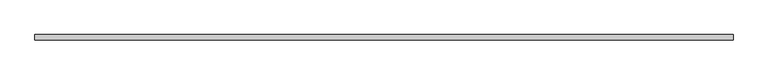
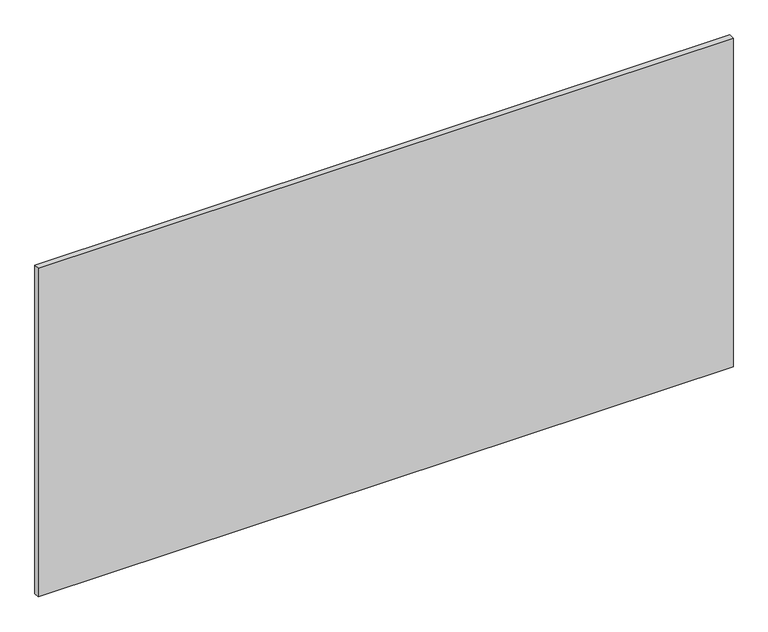
"""IFC4 building model written with IfcOpenShell, lengths in millimetres: proxy geometry, Inner panel:Inner panel:1:Inner panel:1 : Inner panel:Inner panel:300324:300043:Inner panel:1:Inner panel:1 : Inner panel:Inner panel:300324:300043 : Inner panel:Inner panel:1:Inner panel:1 : Inner panel:Inner panel:300324:300043:25 : Inner panel:Inner panel:1:Inner panel:1 : Inner panel:Inner panel:300324:300043:Inner panel:1:Inner panel:1 : Inner panel:Inner panel:300324:300043 : Inner panel:Inner panel:1:Inner panel:1 : Inner panel:Inner panel:300324:300043:300031."""

from ifc_helpers import new_model, si_unit, frame, origin, place, context, project, spatial, polyline, outline, extrude, source, transform, mapped, element, save


def generic_models_4a509fb6(model_context):
    return source(origin(), model_context, "Body", "SweptSolid", [
        extrude(outline(polyline([(592512.5367239, -567913.5913841), (594950.9367239, -567913.5913841), (594950.9367239, -567932.6413841), (592512.5367239, -567932.6413841), (592512.5367239, -567913.5913841)])), frame((0.0, 0.0, 3721.1), z_axis=(0.0, 0.0, 1.0), x_axis=(1.0, 0.0, 0.0)), (0.0, 0.0, 1.0), 1219.2),
    ])


if __name__ == "__main__":
    model = new_model("IFC4")
    model_context = context("Model", 3, world=origin())
    ifc_project = project(units=[si_unit("LENGTHUNIT", "METRE", prefix="MILLI")], contexts=[model_context])
    site = spatial("IfcSite", under=ifc_project)
    building = spatial("IfcBuilding", under=site)
    placement = place(None, origin())
    generic_models_shape = generic_models_4a509fb6(model_context)
    element("IfcBuildingElementProxy", 1, Name="Inner panel:Inner panel:1:Inner panel:1 : Inner panel:Inner panel:300324:300043:Inner panel:1:Inner panel:1 : Inner panel:Inner panel:300324:300043 : Inner panel:Inner panel:1:Inner panel:1 : Inner panel:Inner panel:300324:300043:25 : Inner panel:Inner panel:1:Inner panel:1 : Inner panel:Inner panel:300324:300043:Inner panel:1:Inner panel:1 : Inner panel:Inner panel:300324:300043 : Inner panel:Inner panel:1:Inner panel:1 : Inner panel:Inner panel:300324:300043:300031", ObjectType="Inner panel:Inner panel:1:Inner panel:1 : Inner panel:Inner panel:300324:300043:Inner panel:1:Inner panel:1 : Inner panel:Inner panel:300324:300043 : Inner panel:Inner panel:1:Inner panel:1 : Inner panel:Inner panel:300324:300043:25 : Inner panel:Inner panel:1:Inner panel:1 : Inner panel:Inner panel:300324:300043:Inner panel:1:Inner panel:1 : Inner panel:Inner panel:300324:300043 : Inner panel:Inner panel:1:Inner panel:1 : Inner panel:Inner panel:300324:300043:300031", at=placement, inside=building, context=model_context, shape_type="MappedRepresentation", body=[
        mapped(generic_models_shape, transform((0.0, 0.0, 0.0), x_axis=(1.0, 0.0, 0.0), y_axis=(0.0, 1.0, 0.0), z_axis=(0.0, 0.0, 1.0))),
    ])
    save(model, "model.ifc")

# Revit data of these elements
# Type "Inner panel:Inner panel:1:Inner panel:1 : Inner panel:Inner panel:300324:300043:Inner panel:1:Inner panel:1 : Inner panel:Inner panel:300324:300043 : Inner panel:Inner panel:1:Inner panel:1 : Inner panel:Inner panel:300324:300043:25 : Inner panel:Inner panel:1:Inner panel:1 : Inner panel:Inner panel:300324:300043:Inner panel:1:Inner panel:1 : Inner panel:Inner panel:300324:300043 : Inner panel:Inner panel:1:Inner panel:1 : Inner panel:Inner panel:300324:300043:300031"
#   NameOverride = "Inner panel:Inner panel:1:Inner panel:1 : Inner panel:Inner panel:300324:300043:Inner panel:1:Inner panel:1 : Inner panel:Inner panel:300324:300043 : Inner panel:Inner panel:1:Inner panel:1 : Inner panel:Inner panel:300324:300043:300031"
#   ObjectTypeOverride = "Inner panel:1:Inner panel:1 : Inner panel:Inner panel:300324:300043 : Inner panel:Inner panel:1:Inner panel:1 : Inner panel:Inner panel:300324:300043"
#   Reference = "Inner panel"
#   Tag = "300031"
# Element 1 (IfcBuildingElementProxy, "Inner panel:Inner panel:1:Inner panel:1 : Inner panel:Inner panel:300324:300043:Inner panel:1:Inner panel:1 : Inner panel:Inner panel:300324:300043 : Inner panel:Inner panel:1:Inner panel:1 : Inner panel:Inner panel:300324:300043:25 : Inner panel:Inner panel:1:Inner panel:1 : Inner panel:Inner panel:300324:300043:Inner panel:1:Inner panel:1 : Inner panel:Inner panel:300324:300043 : Inner panel:Inner panel:1:Inner panel:1 : Inner panel:Inner panel:300324:300043:300031")
#   Materials on its faces: "¾” (CLASS A) FIRE RETARDANT PLYWOOD ...OR… IF 1/4\" GYP. BD UNDER PLYWOOD, FLAME SPREAD TO BE CLASS B -  (FINISH: GRADE B - PREFINISHED STAINED/SEALED) - 1/4\" GAP BTWN PANELS (FASTENERS T.B.D.)"
# Materials
#   "¾” (CLASS A) FIRE RETARDANT PLYWOOD ...OR… IF 1/4\" GYP. BD UNDER PLYWOOD, FLAME SPREAD TO BE CLASS B -  (FINISH: GRADE B - PREFINISHED STAINED/SEALED) - 1/4\" GAP BTWN PANELS (FASTENERS T.B.D.)": class "Wood", colour RGB 149 120 74, transparency 0, Description = "Plywood, sheathing grade", Cost = 0
